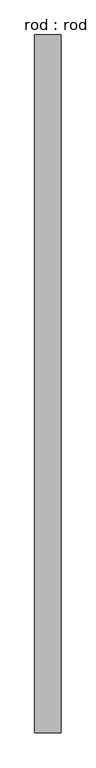
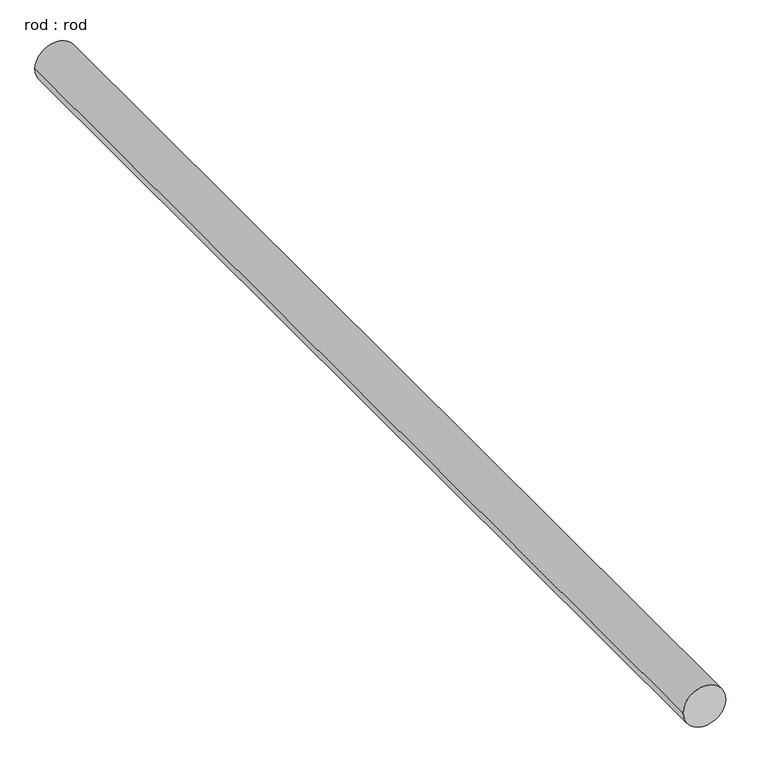
"""IFC4 building model written with IfcOpenShell, lengths in millimetres: proxy geometry, rod : rod."""

import ifcopenshell
import ifcopenshell.guid

model = None  # the IFC model being written
_history = None  # IfcOwnerHistory: only IFC2X3 demands one
_inside = {}  # id of a spatial element -> (the spatial element, [elements in it])
_under = {}  # id of a project, library or spatial element -> (it, [spatial elements below it])
_declared = {}  # id of a project -> (the project, [libraries it declares])
_typed = {}  # id of a type object -> (the type object, [elements of that type])
_made_of = {}  # id of a material, layer set ... -> (it, [elements and type objects made of it])


def new_model(schema):
    """Start an empty IFC model of exactly this schema.

    Asked for "IFC4X3", IfcOpenShell would pick the latest addendum, in which some entities
    have other attributes; the version numbers below select the first issue.
    IFC2X3 requires an IfcOwnerHistory on every rooted entity: one is made here for all.
    """
    global model, _history
    if schema == "IFC4X3":
        model = ifcopenshell.file(schema_version=(4, 3, 0, 0))
    else:
        model = ifcopenshell.file(schema=schema)
    _inside.clear()
    _under.clear()
    _declared.clear()
    _typed.clear()
    _made_of.clear()
    _history = None
    if model.schema == "IFC2X3":
        org = make("IfcOrganization", Name="unknown")
        user = make(
            "IfcPersonAndOrganization",
            ThePerson=make("IfcPerson", FamilyName="unknown"),
            TheOrganization=org,
        )
        app = make(
            "IfcApplication",
            ApplicationDeveloper=org,
            Version="unknown",
            ApplicationFullName="unknown",
            ApplicationIdentifier="unknown",
        )
        _history = make(
            "IfcOwnerHistory",
            OwningUser=user,
            OwningApplication=app,
            ChangeAction="ADDED",
            CreationDate=0,
        )
    return model


def make(cls, **values):
    """One entity of the class cls with the attributes given. An attribute that is None is left unset."""
    return model.create_entity(
        cls, **{name: value for name, value in values.items() if value is not None}
    )


def rooted(cls, **values):
    """An entity with a GlobalId (a new one), such as an element, a storey or a relation."""
    return make(cls, GlobalId=ifcopenshell.guid.new(), OwnerHistory=_history, **values)


def si_unit(unit_type, name, prefix=None):
    """IfcSIUnit, for example si_unit("LENGTHUNIT", "METRE", prefix="MILLI")."""
    return make("IfcSIUnit", UnitType=unit_type, Prefix=prefix, Name=name)


def assignment(units):
    """IfcUnitAssignment: the units of a project."""
    return None if units is None else make("IfcUnitAssignment", Units=units)


def point(xyz):
    """IfcCartesianPoint."""
    return None if xyz is None else make("IfcCartesianPoint", Coordinates=xyz)


def direction(xyz):
    """IfcDirection."""
    return None if xyz is None else make("IfcDirection", DirectionRatios=xyz)


def frame(location, z_axis=None, x_axis=None):
    """IfcAxis2Placement3D, a coordinate frame: its origin and axes. An axis left out is left unset."""
    return make(
        "IfcAxis2Placement3D",
        Location=point(location),
        Axis=direction(z_axis),
        RefDirection=direction(x_axis),
    )


def frame_2d(location, x_axis=None):
    """IfcAxis2Placement2D, a coordinate frame in the plane: its origin and x axis."""
    return make(
        "IfcAxis2Placement2D", Location=point(location), RefDirection=direction(x_axis)
    )


def origin():
    """The frame at (0, 0, 0) with its axes left unset."""
    return frame((0.0, 0.0, 0.0))


def place(relative_to, where):
    """IfcLocalPlacement: puts the frame where relative to a parent placement (None: the world)."""
    return make(
        "IfcLocalPlacement", PlacementRelTo=relative_to, RelativePlacement=where
    )


def context(
    kind, dimensions, precision=None, world=None, true_north=None, identifier=None
):
    """IfcGeometricRepresentationContext, for example the 3D "Model" context."""
    return make(
        "IfcGeometricRepresentationContext",
        ContextIdentifier=identifier,
        ContextType=kind,
        CoordinateSpaceDimension=dimensions,
        Precision=precision,
        WorldCoordinateSystem=world,
        TrueNorth=true_north,
    )


def project(units=None, contexts=None):
    """IfcProject with its units and contexts."""
    return rooted(
        "IfcProject",
        Name="project",
        RepresentationContexts=contexts,
        UnitsInContext=assignment(units),
    )


def spatial(cls, under=None, at=None, **own):
    """A site, building, storey or space (cls), placed at a placement, below another one or the project."""
    s = rooted(cls, ObjectPlacement=at, **own)
    if under is not None:
        _under.setdefault(under.id(), (under, []))[1].append(s)
    return s


def circle_curve(where, radius):
    """IfcCircle in the frame where."""
    return make("IfcCircle", Position=where, Radius=radius)


def trimmed(basis, trim1, trim2, sense, master):
    """IfcTrimmedCurve: the piece of a basis curve between two trims."""
    return make(
        "IfcTrimmedCurve",
        BasisCurve=basis,
        Trim1=trim1,
        Trim2=trim2,
        SenseAgreement=sense,
        MasterRepresentation=master,
    )


def segment(curve, same_sense, transition):
    """IfcCompositeCurveSegment."""
    return make(
        "IfcCompositeCurveSegment",
        Transition=transition,
        SameSense=same_sense,
        ParentCurve=curve,
    )


def composite_curve(segments, self_intersect=None):
    """IfcCompositeCurve: segments joined end to end."""
    return make("IfcCompositeCurve", Segments=segments, SelfIntersect=self_intersect)


def outline(outer, holes=None, kind="AREA"):
    """IfcArbitraryClosedProfileDef: a profile drawn as a closed curve; with holes, ...WithVoids."""
    if holes is None:
        return make("IfcArbitraryClosedProfileDef", ProfileType=kind, OuterCurve=outer)
    return make(
        "IfcArbitraryProfileDefWithVoids",
        ProfileType=kind,
        OuterCurve=outer,
        InnerCurves=holes,
    )


def extrude(swept, where, along, depth):
    """IfcExtrudedAreaSolid: the profile swept, set in the frame where, extruded along a direction by depth."""
    return make(
        "IfcExtrudedAreaSolid",
        SweptArea=swept,
        Position=where,
        ExtrudedDirection=direction(along),
        Depth=depth,
    )


def shape(context_of_items, identifier, shape_type, items):
    """IfcShapeRepresentation: the items that make up one representation, for example the "Body"."""
    return make(
        "IfcShapeRepresentation",
        ContextOfItems=context_of_items,
        RepresentationIdentifier=identifier,
        RepresentationType=shape_type,
        Items=items,
    )


def source(mapping_origin, context_of_items, identifier, shape_type, items):
    """IfcRepresentationMap: a shape defined once, which mapped items show again and again."""
    return make(
        "IfcRepresentationMap",
        MappingOrigin=mapping_origin,
        MappedRepresentation=shape(context_of_items, identifier, shape_type, items),
    )


def transform(
    local_origin,
    x_axis=None,
    y_axis=None,
    z_axis=None,
    scale=None,
    scale2=None,
    scale3=None,
    uniform=True,
):
    """IfcCartesianTransformationOperator3D, or its non-uniform kind. x_axis, y_axis, z_axis: its Axis1, 2, 3."""
    if uniform:
        return make(
            "IfcCartesianTransformationOperator3D",
            Axis1=direction(x_axis),
            Axis2=direction(y_axis),
            LocalOrigin=point(local_origin),
            Scale=scale,
            Axis3=direction(z_axis),
        )
    return make(
        "IfcCartesianTransformationOperator3DnonUniform",
        Axis1=direction(x_axis),
        Axis2=direction(y_axis),
        LocalOrigin=point(local_origin),
        Scale=scale,
        Axis3=direction(z_axis),
        Scale2=scale2,
        Scale3=scale3,
    )


def mapped(mapping_source, mapping_target):
    """IfcMappedItem: shows the shape of a source again, moved by a transform."""
    return make(
        "IfcMappedItem", MappingSource=mapping_source, MappingTarget=mapping_target
    )


def made_of(thing, what):
    """Note that an element or type object is made of a material, layer set ...; save() writes the relation."""
    if what is not None:
        _made_of.setdefault(what.id(), (what, []))[1].append(thing)
    return thing


def element(
    cls,
    number,
    at=None,
    inside=None,
    cuts=None,
    type_object=None,
    material=None,
    context=None,
    identifier="Body",
    shape_type=None,
    held_by="IfcProductDefinitionShape",
    body=None,
    shapes=None,
    **own,
):
    """One element of the class cls, such as IfcWall. Its Tag is "e" and its number.

    at: its placement. inside: the storey or other place that contains it. cuts: it is an
    opening in that element (IfcRelVoidsElement). A single representation is given by context,
    identifier, shape_type and body (its items); several are given by shapes. held_by: the class
    of the entity that holds the representations. save() writes the other relations.
    """
    e = rooted(cls, Tag="e%d" % number, ObjectPlacement=at, **own)
    if body is not None:
        shapes = [shape(context, identifier, shape_type, body)]
    if shapes is not None:
        e.Representation = make(held_by, Representations=shapes)
    if inside is not None:
        _inside.setdefault(inside.id(), (inside, []))[1].append(e)
    if cuts is not None:
        rooted(
            "IfcRelVoidsElement", RelatingBuildingElement=cuts, RelatedOpeningElement=e
        )
    if type_object is not None:
        _typed.setdefault(type_object.id(), (type_object, []))[1].append(e)
    return made_of(e, material)


def aggregate(whole, parts):
    """IfcRelAggregates: a whole, such as a stair, and the parts it consists of."""
    return rooted("IfcRelAggregates", RelatingObject=whole, RelatedObjects=parts)


def save(model, path):
    """Write the relations noted so far, then the file.

    IfcRelAggregates (storeys below a building ...), IfcRelContainedInSpatialStructure (elements
    in a storey), IfcRelDefinesByType, IfcRelAssociatesMaterial and IfcRelDeclares: one each for
    every whole, place, type object, material and project.
    """
    for whole, parts in _under.values():
        aggregate(whole, parts)
    for where, things in _inside.values():
        rooted(
            "IfcRelContainedInSpatialStructure",
            RelatedElements=things,
            RelatingStructure=where,
        )
    for kind, things in _typed.values():
        rooted("IfcRelDefinesByType", RelatedObjects=things, RelatingType=kind)
    for what, things in _made_of.values():
        rooted("IfcRelAssociatesMaterial", RelatedObjects=things, RelatingMaterial=what)
    for by, libraries in _declared.values():
        rooted("IfcRelDeclares", RelatingContext=by, RelatedDefinitions=libraries)
    model.write(path)


def rod_rod_28382057(model_context):
    return source(origin(), model_context, "Body", "SweptSolid", [
        extrude(outline(composite_curve([segment(trimmed(circle_curve(frame_2d((0.0108462, 0.0)), 200.0), [point((0.0108462, 200.0))], [point((0.0108462, -200.0))], False, "CARTESIAN"), True, "CONTINUOUS"), segment(trimmed(circle_curve(frame_2d((0.0108462, 0.0)), 200.0), [point((0.0108462, -200.0))], [point((0.0108462, 200.0))], False, "CARTESIAN"), True, "CONTINUOUS")], self_intersect=False)), frame((0.0, -1212.8269402, 0.0), z_axis=(0.0, 1.0, 0.0), x_axis=(0.0, 0.0, 1.0)), (0.0, 0.0, 1.0), 10611.1111111),
    ])


if __name__ == "__main__":
    model = new_model("IFC4")
    model_context = context("Model", 3, world=origin())
    ifc_project = project(units=[si_unit("LENGTHUNIT", "METRE", prefix="MILLI")], contexts=[model_context])
    site = spatial("IfcSite", under=ifc_project)
    building = spatial("IfcBuilding", under=site)
    placement = place(None, origin())
    rod_rod_shape = rod_rod_28382057(model_context)
    element("IfcBuildingElementProxy", 1, Name="rod : rod", ObjectType="rod : rod", at=placement, inside=building, context=model_context, shape_type="MappedRepresentation", body=[
        mapped(rod_rod_shape, transform((0.0, 0.0, 0.0), x_axis=(1.0, 0.0, 0.0), y_axis=(0.0, 1.0, 0.0), z_axis=(0.0, 0.0, 1.0))),
    ])
    save(model, "model.ifc")

# Revit data of these elements
# Type "rod : rod"
#   Default Elevation = 0
